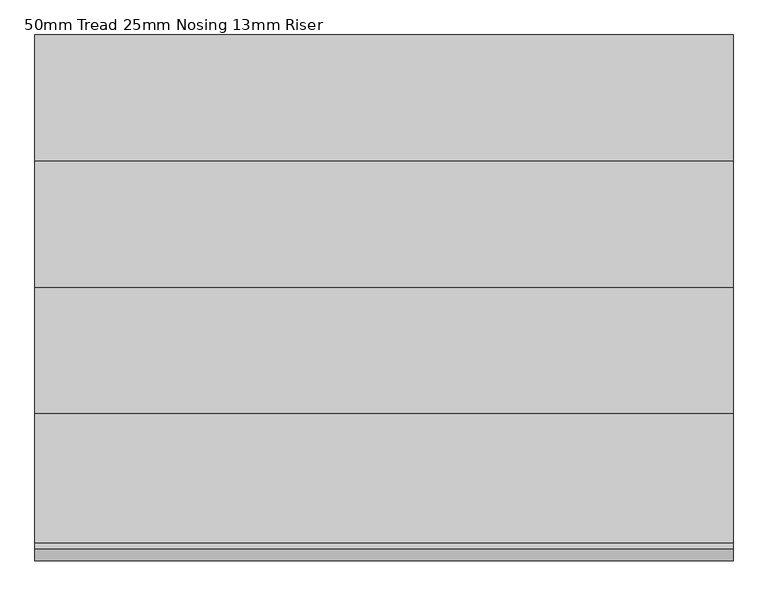
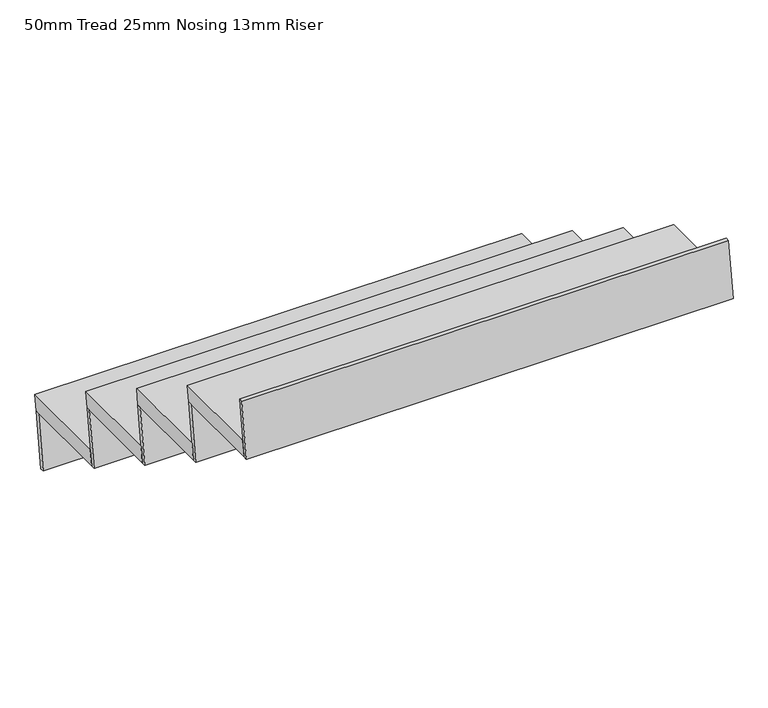
"""IFC4 building model written with IfcOpenShell, lengths in millimetres: stair flight geometry, 50mm Tread 25mm Nosing 13mm Riser."""

from ifc_helpers import new_model, si_unit, frame, origin, place, context, project, spatial, polyline, outline, extrude, source, transform, mapped, element, save


def stair_flight_50mm_tread_25mm_nosing_13mm_riser_b21a55c2(model_context):
    return source(origin(), model_context, "Body", "SweptSolid", [
        extrude(outline(polyline([(7032.4781803, 5794.1176471), (7332.4781803, 5794.1176471), (7325.3948469, 5744.1176471), (7025.3948469, 5744.1176471), (7032.4781803, 5794.1176471)])), frame((-226.7120949, 0.0, 0.0), z_axis=(1.0, 0.0, 0.0), x_axis=(0.0, 1.0, 0.0)), (0.0, 0.0, 1.0), 1520.0),
        extrude(outline(polyline([(7325.3948469, 5744.1176471), (7300.3948469, 5567.6470588), (7287.770036, 5567.6470588), (7312.770036, 5744.1176471), (7325.3948469, 5744.1176471)])), frame((-226.7120949, 0.0, 0.0), z_axis=(1.0, 0.0, 0.0), x_axis=(0.0, 1.0, 0.0)), (0.0, 0.0, 1.0), 1520.0),
        extrude(outline(polyline([(7050.3948469, 5920.5882353), (7025.3948469, 5744.1176471), (7012.770036, 5744.1176471), (7037.770036, 5920.5882353), (7050.3948469, 5920.5882353)])), frame((-226.7120949, 0.0, 0.0), z_axis=(1.0, 0.0, 0.0), x_axis=(0.0, 1.0, 0.0)), (0.0, 0.0, 1.0), 1520.0),
        extrude(outline(polyline([(6757.4781803, 5970.5882353), (7057.4781803, 5970.5882353), (7050.3948469, 5920.5882353), (6750.3948469, 5920.5882353), (6757.4781803, 5970.5882353)])), frame((-226.7120949, 0.0, 0.0), z_axis=(1.0, 0.0, 0.0), x_axis=(0.0, 1.0, 0.0)), (0.0, 0.0, 1.0), 1520.0),
        extrude(outline(polyline([(6775.3948469, 6097.0588235), (6750.3948469, 5920.5882353), (6737.770036, 5920.5882353), (6762.770036, 6097.0588235), (6775.3948469, 6097.0588235)])), frame((-226.7120949, 0.0, 0.0), z_axis=(1.0, 0.0, 0.0), x_axis=(0.0, 1.0, 0.0)), (0.0, 0.0, 1.0), 1520.0),
        extrude(outline(polyline([(6482.4781803, 6147.0588235), (6782.4781803, 6147.0588235), (6775.3948469, 6097.0588235), (6475.3948469, 6097.0588235), (6482.4781803, 6147.0588235)])), frame((-226.7120949, 0.0, 0.0), z_axis=(1.0, 0.0, 0.0), x_axis=(0.0, 1.0, 0.0)), (0.0, 0.0, 1.0), 1520.0),
        extrude(outline(polyline([(6500.3948469, 6273.5294118), (6475.3948469, 6097.0588235), (6462.770036, 6097.0588235), (6487.770036, 6273.5294118), (6500.3948469, 6273.5294118)])), frame((-226.7120949, 0.0, 0.0), z_axis=(1.0, 0.0, 0.0), x_axis=(0.0, 1.0, 0.0)), (0.0, 0.0, 1.0), 1520.0),
        extrude(outline(polyline([(6225.3948469, 6450.0), (6200.3948469, 6273.5294118), (6187.770036, 6273.5294118), (6212.770036, 6450.0), (6225.3948469, 6450.0)])), frame((-226.7120949, 0.0, 0.0), z_axis=(1.0, 0.0, 0.0), x_axis=(0.0, 1.0, 0.0)), (0.0, 0.0, 1.0), 1520.0),
        extrude(outline(polyline([(6207.4781803, 6323.5294118), (6507.4781803, 6323.5294118), (6500.3948469, 6273.5294118), (6200.3948469, 6273.5294118), (6207.4781803, 6323.5294118)])), frame((-226.7120949, 0.0, 0.0), z_axis=(1.0, 0.0, 0.0), x_axis=(0.0, 1.0, 0.0)), (0.0, 0.0, 1.0), 1520.0),
    ])


if __name__ == "__main__":
    model = new_model("IFC4")
    model_context = context("Model", 3, world=origin())
    ifc_project = project(units=[si_unit("LENGTHUNIT", "METRE", prefix="MILLI")], contexts=[model_context])
    site = spatial("IfcSite", under=ifc_project)
    building = spatial("IfcBuilding", under=site)
    placement = place(None, origin())
    stair_flight_50mm_tread_25mm_nosing_13mm_riser_shape = stair_flight_50mm_tread_25mm_nosing_13mm_riser_b21a55c2(model_context)
    element("IfcStairFlight", 1, ObjectType="50mm Tread 25mm Nosing 13mm Riser", at=placement, inside=building, context=model_context, shape_type="MappedRepresentation", body=[
        mapped(stair_flight_50mm_tread_25mm_nosing_13mm_riser_shape, transform((0.0, 0.0, 0.0), x_axis=(1.0, 0.0, 0.0), y_axis=(0.0, 1.0, 0.0), z_axis=(0.0, 0.0, 1.0))),
    ])
    save(model, "model.ifc")
